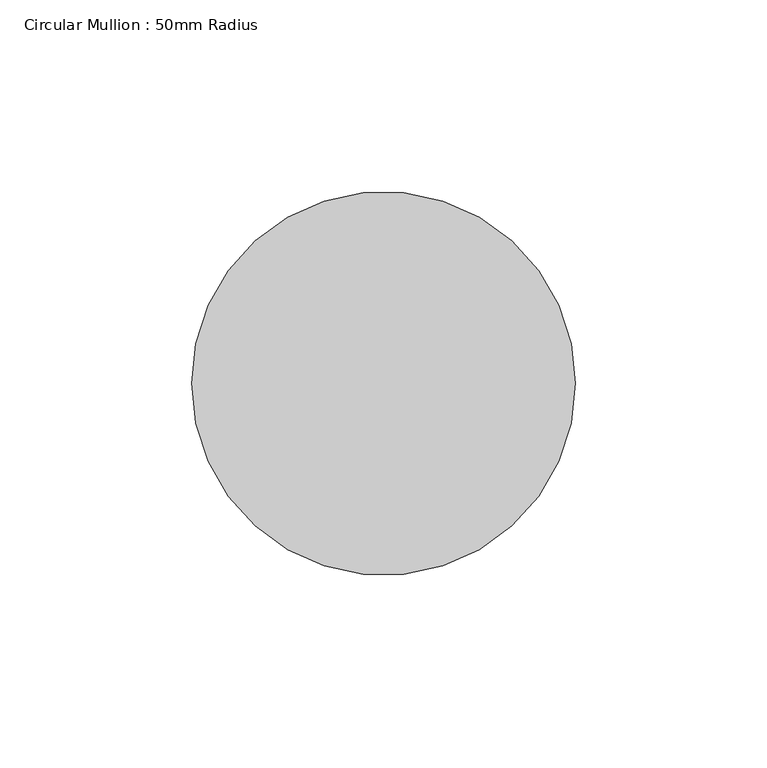
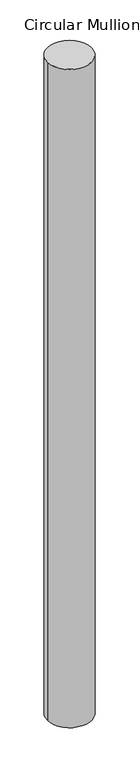
"""IFC4 building model written with IfcOpenShell, lengths in millimetres: member geometry, Circular Mullion : 50mm Radius."""

from ifc_helpers import new_model, si_unit, point, frame, origin, origin_2d, place, context, project, spatial, circle_curve, trimmed, segment, composite_curve, outline, extrude, source, transform, mapped, element, save


def circular_mullion_50mm_radius_1e7c025b(model_context):
    return source(origin(), model_context, "Body", "SweptSolid", [
        extrude(outline(composite_curve([segment(trimmed(circle_curve(origin_2d(), 50.0), [point((50.0, 0.0))], [point((-50.0, 0.0))], False, "CARTESIAN"), True, "CONTINUOUS"), segment(trimmed(circle_curve(origin_2d(), 50.0), [point((-50.0, 0.0))], [point((50.0, 0.0))], False, "CARTESIAN"), True, "CONTINUOUS")], self_intersect=False)), frame((0.0, 0.0, -1576.2891218), z_axis=(0.0, 0.0, 1.0), x_axis=(1.0, 0.0, 0.0)), (0.0, 0.0, 1.0), 1576.2891218),
    ])


if __name__ == "__main__":
    model = new_model("IFC4")
    model_context = context("Model", 3, world=origin())
    ifc_project = project(units=[si_unit("LENGTHUNIT", "METRE", prefix="MILLI")], contexts=[model_context])
    site = spatial("IfcSite", under=ifc_project)
    building = spatial("IfcBuilding", under=site)
    placement = place(None, origin())
    circular_mullion_50mm_radius_shape = circular_mullion_50mm_radius_1e7c025b(model_context)
    element("IfcMember", 1, ObjectType="Circular Mullion : 50mm Radius", at=placement, inside=building, context=model_context, shape_type="MappedRepresentation", body=[
        mapped(circular_mullion_50mm_radius_shape, transform((0.0, 0.0, 0.0), x_axis=(1.0, 0.0, 0.0), y_axis=(0.0, 1.0, 0.0), z_axis=(0.0, 0.0, 1.0))),
    ])
    save(model, "model.ifc")

# Revit data of these elements
# Type "Circular Mullion : 50mm Radius"
#   built-in parameter 1007350 = 0.164042 (stored number, unit not read)
# Element 1 (IfcMember, "Circular Mullion : 50mm Radius")
#   Materials on its faces: "Aluminium"
# Materials
#   "Aluminium": class "Metal", colour RGB 247 247 247, transparency 0, Description = "Aluminium 6061", Cost = 0
